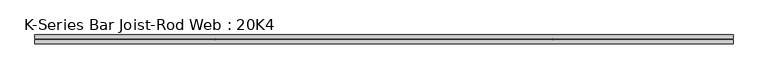
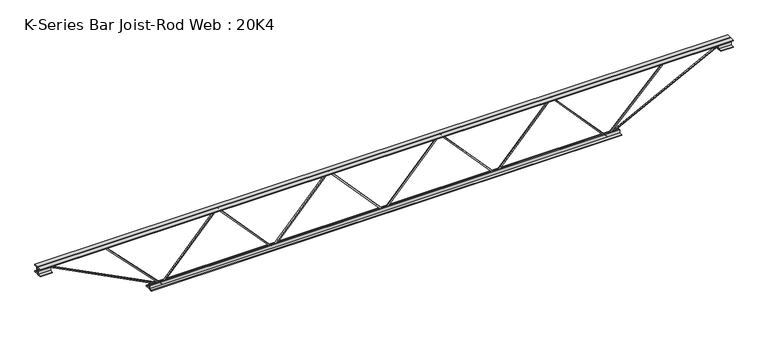
"""IFC4 building model written with IfcOpenShell, lengths in millimetres: beam geometry, K-Series Bar Joist-Rod Web : 20K4."""

from ifc_helpers import new_model, si_unit, frame, origin, place, context, project, spatial, polyline, outline, extrude, source, transform, mapped, element, save


def k_series_bar_joist_rod_web_20k4_fb802784(model_context):
    return source(origin(), model_context, "Body", "SweptSolid", [
        extrude(outline(polyline([(-242.8875, 0.0), (-252.4125, 0.0), (-252.4125, 5.279971), (242.8875, 456.129971), (242.8875, 458.270029), (-252.4125, 909.120029), (-252.4125, 914.4), (-242.8875, 914.4), (-242.8875, 913.329971), (252.4125, 462.479971), (252.4125, 451.920029), (-242.8875, 1.070029), (-242.8875, 0.0)])), frame((0.0, -4.7625, 0.0), z_axis=(0.0, 1.0, 0.0), x_axis=(0.0, 0.0, 1.0)), (0.0, 0.0, 1.0), 9.525),
        extrude(outline(polyline([(-242.8875, -914.4), (-252.4125, -914.4), (-252.4125, -909.120029), (242.8875, -458.270029), (242.8875, -456.129971), (-252.4125, -5.279971), (-252.4125, 0.0), (-242.8875, 0.0), (-242.8875, -1.070029), (252.4125, -451.920029), (252.4125, -462.479971), (-242.8875, -913.329971), (-242.8875, -914.4)])), frame((0.0, -4.7625, 0.0), z_axis=(0.0, 1.0, 0.0), x_axis=(0.0, 0.0, 1.0)), (0.0, 0.0, 1.0), 9.525),
        extrude(outline(polyline([(-242.8875, 914.4), (-252.4125, 914.4), (-252.4125, 919.679971), (242.8875, 1370.529971), (242.8875, 1372.670029), (-252.4125, 1823.520029), (-252.4125, 1828.8), (-242.8875, 1828.8), (-242.8875, 1827.729971), (252.4125, 1376.879971), (252.4125, 1366.320029), (-242.8875, 915.470029), (-242.8875, 914.4)])), frame((0.0, -4.7625, 0.0), z_axis=(0.0, 1.0, 0.0), x_axis=(0.0, 0.0, 1.0)), (0.0, 0.0, 1.0), 9.525),
        extrude(outline(polyline([(-242.8875, -1828.8), (-252.4125, -1828.8), (-252.4125, -1823.520029), (242.8875, -1372.670029), (242.8875, -1370.529971), (-252.4125, -919.679971), (-252.4125, -914.4), (-242.8875, -914.4), (-242.8875, -915.470029), (252.4125, -1366.320029), (252.4125, -1376.879971), (-242.8875, -1827.729971), (-242.8875, -1828.8)])), frame((0.0, -4.7625, 0.0), z_axis=(0.0, 1.0, 0.0), x_axis=(0.0, 0.0, 1.0)), (0.0, 0.0, 1.0), 9.525),
        extrude(outline(polyline([(4.7625, 254.0), (36.5125, 254.0), (36.5125, 247.65), (11.1125, 247.65), (11.1125, 222.25), (4.7625, 222.25), (4.7625, 254.0)])), frame((-2844.8, 0.0, 0.0), z_axis=(1.0, 0.0, 0.0), x_axis=(0.0, 1.0, 0.0)), (0.0, 0.0, 1.0), 5689.6),
        extrude(outline(polyline([(-4.7625, 254.0), (-4.7625, 222.25), (-11.1125, 222.25), (-11.1125, 247.65), (-36.5125, 247.65), (-36.5125, 254.0), (-4.7625, 254.0)])), frame((-2844.8, 0.0, 0.0), z_axis=(1.0, 0.0, 0.0), x_axis=(0.0, 1.0, 0.0)), (0.0, 0.0, 1.0), 5689.6),
        extrude(outline(polyline([(-4.7625, 190.5), (-36.5125, 190.5), (-36.5125, 196.85), (-11.1125, 196.85), (-11.1125, 222.25), (-4.7625, 222.25), (-4.7625, 190.5)])), frame((-2844.8, 0.0, 0.0), z_axis=(1.0, 0.0, 0.0), x_axis=(0.0, 1.0, 0.0)), (0.0, 0.0, 1.0), 101.6),
        extrude(outline(polyline([(36.5125, 190.5), (4.7625, 190.5), (4.7625, 222.25), (11.1125, 222.25), (11.1125, 196.85), (36.5125, 196.85), (36.5125, 190.5)])), frame((-2844.8, 0.0, 0.0), z_axis=(1.0, 0.0, 0.0), x_axis=(0.0, 1.0, 0.0)), (0.0, 0.0, 1.0), 101.6),
        extrude(outline(polyline([(4.7625, 190.5), (4.7625, 222.25), (11.1125, 222.25), (11.1125, 196.85), (36.5125, 196.85), (36.5125, 190.5), (4.7625, 190.5)])), frame((2743.2, 0.0, 0.0), z_axis=(1.0, 0.0, 0.0), x_axis=(0.0, 1.0, 0.0)), (0.0, 0.0, 1.0), 101.6),
        extrude(outline(polyline([(-4.7625, 190.5), (-36.5125, 190.5), (-36.5125, 196.85), (-11.1125, 196.85), (-11.1125, 222.25), (-4.7625, 222.25), (-4.7625, 190.5)])), frame((2743.2, 0.0, 0.0), z_axis=(1.0, 0.0, 0.0), x_axis=(0.0, 1.0, 0.0)), (0.0, 0.0, 1.0), 101.6),
        extrude(outline(polyline([(4.7625, -254.0), (4.7625, -222.25), (11.1125, -222.25), (11.1125, -247.65), (36.5125, -247.65), (36.5125, -254.0), (4.7625, -254.0)])), frame((-1930.4, 0.0, 0.0), z_axis=(1.0, 0.0, 0.0), x_axis=(0.0, 1.0, 0.0)), (0.0, 0.0, 1.0), 3860.8),
        extrude(outline(polyline([(-4.7625, -254.0), (-36.5125, -254.0), (-36.5125, -247.65), (-11.1125, -247.65), (-11.1125, -222.25), (-4.7625, -222.25), (-4.7625, -254.0)])), frame((-1930.4, 0.0, 0.0), z_axis=(1.0, 0.0, 0.0), x_axis=(0.0, 1.0, 0.0)), (0.0, 0.0, 1.0), 3860.8),
        extrude(outline(polyline([(0.0, -9.525), (0.0, 0.0), (1028.0726482, 0.0), (1028.0726482, -9.525), (0.0, -9.525)])), frame((-2745.3767905, 4.7625, 218.0140834), z_axis=(0.45706886650213807, 0.0, 0.8894313077885502), x_axis=(0.8894313077885502, 0.0, -0.45706886650213807)), (0.0, 0.0, 1.0), 9.525),
        extrude(outline(polyline([(4.7625, 4.7625), (4.7625, -4.7625), (-4.7625, -4.7625), (-4.7625, 4.7625), (4.7625, 4.7625)])), frame((-1828.8, 0.0, -247.65), z_axis=(-0.697354959803679, 0.0, 0.7167259309088861), x_axis=(0.0, -1.0, 0.0)), (0.0, 0.0, 1.0), 655.6202026),
        extrude(outline(polyline([(0.0, -9.525), (0.0, 0.0), (1028.0726482, 0.0), (1028.0726482, -9.525), (0.0, -9.525)])), frame((2745.3767905, -4.7625, 218.0140834), z_axis=(-0.45706886650212714, 0.0, 0.8894313077885558), x_axis=(-0.8894313077885558, 0.0, -0.45706886650212714)), (0.0, 0.0, 1.0), 9.525),
        extrude(outline(polyline([(4.7625, 4.7625), (4.7625, -4.7625), (-4.7625, -4.7625), (-4.7625, 4.7625), (4.7625, 4.7625)])), frame((1828.8, 0.0, -247.65), z_axis=(0.6973549598036842, 0.0, 0.716725930908881), x_axis=(0.0, -1.0, 0.0)), (0.0, 0.0, 1.0), 655.6202026),
    ])


if __name__ == "__main__":
    model = new_model("IFC4")
    model_context = context("Model", 3, world=origin())
    ifc_project = project(units=[si_unit("LENGTHUNIT", "METRE", prefix="MILLI")], contexts=[model_context])
    site = spatial("IfcSite", under=ifc_project)
    building = spatial("IfcBuilding", under=site)
    placement = place(None, origin())
    k_series_bar_joist_rod_web_20k4_shape = k_series_bar_joist_rod_web_20k4_fb802784(model_context)
    element("IfcBeam", 1, ObjectType="K-Series Bar Joist-Rod Web : 20K4", at=placement, inside=building, context=model_context, shape_type="MappedRepresentation", body=[
        mapped(k_series_bar_joist_rod_web_20k4_shape, transform((0.0, 0.0, 0.0), x_axis=(1.0, 0.0, 0.0), y_axis=(0.0, 1.0, 0.0), z_axis=(0.0, 0.0, 1.0))),
    ])
    save(model, "model.ifc")

# Revit data of these elements
# Type "K-Series Bar Joist-Rod Web : 20K4"
#   Assembly Code = "B1010350"
#   Wt = 7.6
#   Web Thickness = 0' - 0 3/8"
#   Start Offset [instance default] = 0' - 0"
#   Start Extension [instance default] = 0' - 0"
#   Seat Length = 0' - 4"
#   Seat Depth = 0' - 2 1/2"
#   PanelArrayLength [instance default] = 17' - 4"
#   Panel [instance default] = 3' - 5.6"
#   End Offset [instance default] = 0' - 0"
#   End Extension [instance default] = 0' - 0"
#   End Panel = 3' - 4"
#   Cord Leg = 0' - 1 1/4"
#   Chord Thickness = 0' - 0 1/4"
#   Length [instance default] = 24' - 0"
#   Depth = 1' - 8"
#   PanelArrayNum [instance default] = 5
#   Structural Material = none
# Element 1 (IfcBeam, "K-Series Bar Joist-Rod Web : 20K4")
#   PanelArrayLength = 12' - 0"
#   Panel = 3' - 0"
#   PanelArrayNum = 4
